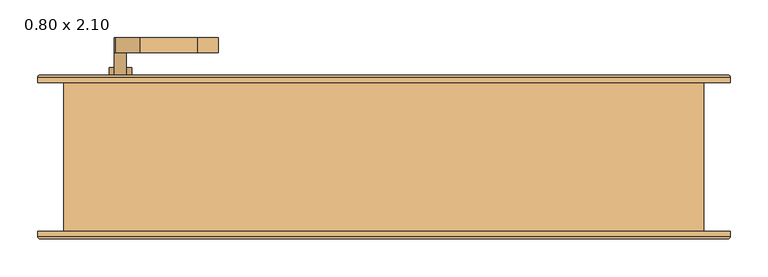
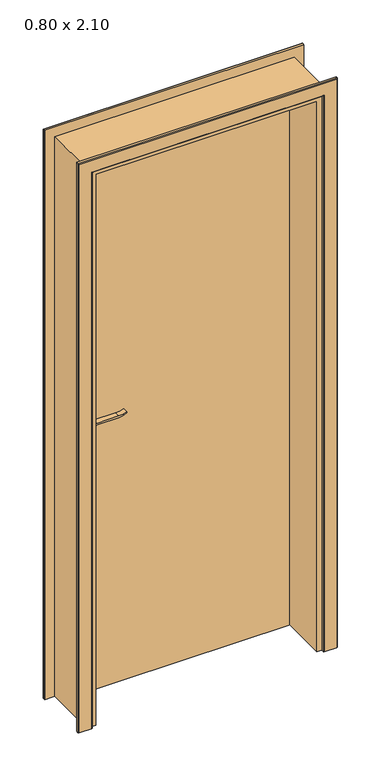
"""IFC4 building model written with IfcOpenShell, lengths in millimetres: door geometry, .CC_ND 300_PORTA SIMPLES DE ABRIR_COM EXTENSÃO : 0.80 x 2.10."""

from ifc_helpers import new_model, si_unit, point, frame, frame_2d, origin, origin_with_axes, place, context, project, spatial, polyline, circle_curve, ellipse_curve, trimmed, segment, composite_curve, outline, extrude, faceted_brep, source, transform, mapped, element, save
from ifc_brep_helpers import plane_surface, cylinder_surface, advanced_brep


def door_0_80_x_2_10_6188e507(model_context):
    return source(origin(), model_context, "Body", "SolidModel", [
        extrude(outline(composite_curve([segment(trimmed(circle_curve(frame_2d((964.5, -350.0)), 15.0), [point((964.5, -335.0))], [point((964.5, -365.0))], False, "CARTESIAN"), True, "CONTINUOUS"), segment(trimmed(circle_curve(frame_2d((964.5, -350.0)), 15.0), [point((964.5, -365.0))], [point((964.5, -335.0))], False, "CARTESIAN"), True, "CONTINUOUS")], self_intersect=False)), frame((0.0, 108.8, 0.0), z_axis=(0.0, 1.0, 0.0), x_axis=(0.0, 0.0, 1.0)), (0.0, 0.0, 1.0), 10.0),
        extrude(outline(composite_curve([segment(trimmed(circle_curve(frame_2d((964.5, -350.0)), 15.0), [point((964.5, -335.0))], [point((964.5, -365.0))], False, "CARTESIAN"), True, "CONTINUOUS"), segment(trimmed(circle_curve(frame_2d((964.5, -350.0)), 15.0), [point((964.5, -365.0))], [point((964.5, -335.0))], False, "CARTESIAN"), True, "CONTINUOUS")], self_intersect=False)), frame((0.0, 48.8, 0.0), z_axis=(0.0, 1.0, 0.0), x_axis=(0.0, 0.0, 1.0)), (0.0, 0.0, 1.0), 10.0),
        extrude(outline(composite_curve([segment(trimmed(circle_curve(frame_2d((1024.5, -350.0)), 8.0), [point((1029.1523287, -356.5081363))], [point((1024.5, -342.0))], False, "CARTESIAN"), True, "CONTINUOUS"), segment(trimmed(circle_curve(frame_2d((1019.3738613, -324.6138099)), 18.1261387), [point((1024.5, -342.0))], [point((1037.5, -324.6138099))], True, "CARTESIAN"), True, "CONTINUOUS"), segment(polyline([(1037.5, -324.6138099), (1037.5, -248.3564091)]), True, "CONTINUOUS"), segment(trimmed(circle_curve(frame_2d((1096.7709207, -251.9396612)), 59.3791355), [point((1037.5, -248.3564091))], [point((1046.7135558, -220.0))], False, "CARTESIAN"), True, "CONTINUOUS"), segment(polyline([(1046.7135558, -220.0), (1049.5, -220.0)]), True, "CONTINUOUS"), segment(trimmed(circle_curve(frame_2d((1127.7850638, -248.4227909)), 83.2850902), [point((1049.5, -220.0))], [point((1044.5, -248.3564091))], True, "CARTESIAN"), True, "CONTINUOUS"), segment(polyline([(1044.5, -248.3564091), (1044.5, -324.6325667)]), True, "CONTINUOUS"), segment(trimmed(circle_curve(frame_2d((1007.2555521, -326.3324871)), 37.2832219), [point((1044.5, -324.6325667))], [point((1029.1523287, -356.5081363))], False, "CARTESIAN"), True, "CONTINUOUS")], self_intersect=False)), frame((0.0, 138.8, 0.0), z_axis=(0.0, 1.0, 0.0), x_axis=(0.0, 0.0, 1.0)), (0.0, 0.0, 1.0), 20.0),
        extrude(outline(composite_curve([segment(trimmed(circle_curve(frame_2d((1019.3738682, -324.6138122)), 18.1261318), [point((1024.4999903, -342.0))], [point((1037.5, -324.6138122))], True, "CARTESIAN"), True, "CONTINUOUS"), segment(polyline([(1037.5, -324.6138122), (1037.5, -248.3564091)]), True, "CONTINUOUS"), segment(trimmed(circle_curve(frame_2d((1096.7709207, -251.9396612)), 59.3791355), [point((1037.5, -248.3564091))], [point((1046.7135558, -220.0))], False, "CARTESIAN"), True, "CONTINUOUS"), segment(polyline([(1046.7135558, -220.0), (1049.5, -220.0)]), True, "CONTINUOUS"), segment(trimmed(circle_curve(frame_2d((1127.7850638, -248.4227909)), 83.2850902), [point((1049.5, -220.0))], [point((1044.5, -248.3564091))], True, "CARTESIAN"), True, "CONTINUOUS"), segment(polyline([(1044.5, -248.3564091), (1044.5, -324.6325667)]), True, "CONTINUOUS"), segment(trimmed(circle_curve(frame_2d((1007.2555521, -326.3324871)), 37.2832219), [point((1044.5, -324.6325667))], [point((1029.1523287, -356.5081363))], False, "CARTESIAN"), True, "CONTINUOUS"), segment(trimmed(circle_curve(frame_2d((1024.5, -350.0)), 8.0), [point((1029.1523287, -356.5081363))], [point((1024.4999903, -342.0))], False, "CARTESIAN"), True, "CONTINUOUS")], self_intersect=False)), frame((0.0, 8.8, 0.0), z_axis=(0.0, 1.0, 0.0), x_axis=(0.0, 0.0, 1.0)), (0.0, 0.0, 1.0), 20.0),
        extrude(outline(composite_curve([segment(trimmed(circle_curve(frame_2d((1024.5, -350.0)), 8.0), [point((1024.5, -342.0))], [point((1024.5, -358.0))], False, "CARTESIAN"), True, "CONTINUOUS"), segment(trimmed(circle_curve(frame_2d((1024.5, -350.0)), 8.0), [point((1024.5, -358.0))], [point((1024.5, -342.0))], False, "CARTESIAN"), True, "CONTINUOUS")], self_intersect=False)), frame((0.0, 108.8, 0.0), z_axis=(0.0, 1.0, 0.0), x_axis=(0.0, 0.0, 1.0)), (0.0, 0.0, 1.0), 30.0),
        extrude(outline(composite_curve([segment(trimmed(circle_curve(frame_2d((1024.5, -350.0)), 8.0), [point((1024.5, -342.0))], [point((1024.5, -358.0))], False, "CARTESIAN"), True, "CONTINUOUS"), segment(trimmed(circle_curve(frame_2d((1024.5, -350.0)), 8.0), [point((1024.5, -358.0))], [point((1024.5, -342.0))], False, "CARTESIAN"), True, "CONTINUOUS")], self_intersect=False)), frame((0.0, 28.8, 0.0), z_axis=(0.0, 1.0, 0.0), x_axis=(0.0, 0.0, 1.0)), (0.0, 0.0, 1.0), 30.0),
        extrude(outline(composite_curve([segment(trimmed(circle_curve(frame_2d((954.5, -350.0)), 25.0), [point((954.5, -375.0))], [point((954.5, -325.0))], False, "CARTESIAN"), True, "CONTINUOUS"), segment(polyline([(954.5, -325.0), (1024.5, -325.0)]), True, "CONTINUOUS"), segment(trimmed(circle_curve(frame_2d((1024.5, -350.0)), 25.0), [point((1024.5, -325.0))], [point((1024.5, -375.0))], False, "CARTESIAN"), True, "CONTINUOUS"), segment(polyline([(1024.5, -375.0), (954.5, -375.0)]), True, "CONTINUOUS")], self_intersect=False)), frame((0.0, 98.8, 0.0), z_axis=(0.0, 1.0, 0.0), x_axis=(0.0, 0.0, 1.0)), (0.0, 0.0, 1.0), 10.0),
        extrude(outline(composite_curve([segment(trimmed(circle_curve(frame_2d((954.5, -350.0)), 25.0), [point((954.5, -375.0))], [point((954.5, -325.0))], False, "CARTESIAN"), True, "CONTINUOUS"), segment(polyline([(954.5, -325.0), (1024.5, -325.0)]), True, "CONTINUOUS"), segment(trimmed(circle_curve(frame_2d((1024.5, -350.0)), 25.0), [point((1024.5, -325.0))], [point((1024.5, -375.0))], False, "CARTESIAN"), True, "CONTINUOUS"), segment(polyline([(1024.5, -375.0), (954.5, -375.0)]), True, "CONTINUOUS")], self_intersect=False)), frame((0.0, 58.8, 0.0), z_axis=(0.0, 1.0, 0.0), x_axis=(0.0, 0.0, 1.0)), (0.0, 0.0, 1.0), 10.0),
        advanced_brep(
        [(-460.0, 98.8, 0.0), (-460.0, 105.8, 0.0), (-457.0, 108.8, 0.0), (-413.0, 108.8, 0.0), (-410.0, 105.8, 0.0), (-410.0, 98.8, 0.0), (-410.0, 98.8, 2085.0), (410.0, 98.8, 2085.0), (410.0, 98.8, 0.0), (460.0, 98.8, 0.0), (460.0, 98.8, 2135.0), (-460.0, 98.8, 2135.0), (-410.0, 105.8, 2085.0), (-413.0, 108.8, 2088.0), (-457.0, 108.8, 2132.0), (457.0, 108.8, 2132.0), (457.0, 108.8, 0.0), (413.0, 108.8, 0.0), (413.0, 108.8, 2088.0), (-460.0, 105.8, 2135.0), (460.0, 105.8, 0.0), (460.0, 105.8, 2135.0), (410.0, 105.8, 0.0), (410.0, 105.8, 2085.0)],
        [
            (0, 1),
            (1, 2, circle_curve(frame((-457.0, 105.8, 0.0), z_axis=(0.0, 0.0, -1.0), x_axis=(1.0, 0.0, 0.0)), 3.0)),
            (2, 3),
            (3, 4, circle_curve(frame((-413.0, 105.8, 0.0), z_axis=(0.0, 0.0, -1.0), x_axis=(1.0, 0.0, 0.0)), 3.0)),
            (4, 5),
            (5, 0),
            (5, 6),
            (6, 7),
            (7, 8),
            (8, 9),
            (9, 10),
            (10, 11),
            (11, 0),
            (4, 12),
            (12, 6),
            (3, 13),
            (13, 12, ellipse_curve(frame((-413.0, 105.8, 2088.0), z_axis=(-0.7071067811865475, 0.0, -0.7071067811865475), x_axis=(0.7071067811865474, 0.0, -0.7071067811865476)), 4.2426407, 3.0)),
            (2, 14),
            (14, 15),
            (15, 16),
            (16, 17),
            (17, 18),
            (18, 13),
            (1, 19),
            (19, 14, ellipse_curve(frame((-457.0, 105.8, 2132.0), z_axis=(-0.7071067811865475, 0.0, -0.7071067811865475), x_axis=(0.7071067811865474, 0.0, -0.7071067811865476)), 4.2426407, 3.0)),
            (11, 19),
            (9, 20),
            (20, 21),
            (21, 10),
            (8, 22),
            (22, 17, circle_curve(frame((413.0, 105.8, 0.0), z_axis=(0.0, 0.0, -1.0), x_axis=(-1.0, 0.0, 0.0)), 3.0)),
            (16, 20, circle_curve(frame((457.0, 105.8, 0.0), z_axis=(0.0, 0.0, -1.0), x_axis=(-1.0, 0.0, 0.0)), 3.0)),
            (23, 22),
            (7, 23),
            (23, 18, ellipse_curve(frame((413.0, 105.8, 2088.0), z_axis=(0.7071067811865475, 0.0, -0.7071067811865475), x_axis=(0.7071067811865474, 0.0, 0.7071067811865476)), 4.2426407, 3.0)),
            (15, 21, ellipse_curve(frame((457.0, 105.8, 2132.0), z_axis=(0.7071067811865475, 0.0, -0.7071067811865475), x_axis=(0.7071067811865474, 0.0, 0.7071067811865476)), 4.2426407, 3.0)),
            (12, 23),
            (21, 19),
        ],
        [
            plane_surface(frame((-410.0, 98.8, 0.0), z_axis=(0.0, 0.0, -1.0), x_axis=(0.0, -1.0, 0.0))),
            plane_surface(frame((-460.0, 98.8, 0.0), z_axis=(0.0, -1.0, 0.0), x_axis=(0.0, 0.0, 1.0))),
            plane_surface(frame((-410.0, 98.8, 0.0), z_axis=(1.0, 0.0, 0.0), x_axis=(0.0, 0.0, 1.0))),
            cylinder_surface(frame((-413.0, 105.8, 0.0), z_axis=(0.0, 0.0, -1.0), x_axis=(1.0, 0.0, 0.0)), 3.0),
            plane_surface(frame((-413.0, 108.8, 0.0), z_axis=(0.0, 1.0, 0.0), x_axis=(0.0, 0.0, 1.0))),
            cylinder_surface(frame((-457.0, 105.8, 0.0), z_axis=(0.0, 0.0, -1.0), x_axis=(1.0, 0.0, 0.0)), 3.0),
            plane_surface(frame((-460.0, 105.8, 0.0), z_axis=(-1.0, 0.0, 0.0), x_axis=(0.0, 0.0, 1.0))),
            plane_surface(frame((460.0, 105.8, 2135.0), z_axis=(1.0, 0.0, 0.0), x_axis=(0.0, 0.0, -1.0))),
            plane_surface(frame((410.0, 98.8, 0.0), z_axis=(0.0, 0.0, -1.0), x_axis=(0.0, -1.0, 0.0))),
            plane_surface(frame((410.0, 98.8, 2085.0), z_axis=(-1.0, 0.0, 0.0), x_axis=(0.0, 0.0, -1.0))),
            cylinder_surface(frame((413.0, 105.8, 2085.0), z_axis=(0.0, 0.0, 1.0), x_axis=(-1.0, 0.0, 0.0)), 3.0),
            cylinder_surface(frame((457.0, 105.8, 2085.0), z_axis=(0.0, 0.0, 1.0), x_axis=(-1.0, 0.0, 0.0)), 3.0),
            plane_surface(frame((-410.0, 98.8, 2085.0), z_axis=(0.0, 0.0, -1.0), x_axis=(1.0, 0.0, 0.0))),
            plane_surface(frame((-460.0, 105.8, 2135.0), z_axis=(0.0, 0.0, 1.0), x_axis=(1.0, 0.0, 0.0))),
            cylinder_surface(frame((-410.0, 105.8, 2088.0), z_axis=(-1.0, 0.0, 0.0), x_axis=(0.0, 0.0, -1.0)), 3.0),
            cylinder_surface(frame((-410.0, 105.8, 2132.0), z_axis=(-1.0, 0.0, 0.0), x_axis=(0.0, 0.0, -1.0)), 3.0),
        ],
        [
            (0, [[1, 2, 3, 4, 5, 6]]),
            (1, [[7, 8, 9, 10, 11, 12, 13, -6]]),
            (2, [[14, 15, -7, -5]]),
            (3, [[16, 17, -14, -4]]),
            (4, [[18, 19, 20, 21, 22, 23, -16, -3]]),
            (5, [[24, 25, -18, -2]]),
            (6, [[-13, 26, -24, -1]]),
            (7, [[-11, 27, 28, 29]]),
            (8, [[-10, 30, 31, -21, 32, -27]]),
            (9, [[33, -30, -9, 34]]),
            (10, [[-22, -31, -33, 35]]),
            (11, [[-28, -32, -20, 36]]),
            (12, [[37, -34, -8, -15]]),
            (13, [[-12, -29, 38, -26]]),
            (14, [[-23, -35, -37, -17]]),
            (15, [[-38, -36, -19, -25]]),
        ],
    ),
        advanced_brep(
        [(460.0, -98.8, 0.0), (460.0, -105.8342217, 0.0), (457.0342217, -108.8, 0.0), (412.9842717, -108.8, 0.0), (410.0, -105.8157283, 0.0), (410.0, -98.8, 0.0), (410.0, -98.8, 2085.0), (-410.0, -98.8, 2085.0), (-410.0, -98.8, 0.0), (-460.0, -98.8, 0.0), (-460.0, -98.8, 2135.0), (460.0, -98.8, 2135.0), (410.0, -105.8157283, 2085.0), (412.9842717, -108.8, 2087.9842717), (457.0342217, -108.8, 2132.0342217), (-457.0342217, -108.8, 2132.0342217), (-457.0342217, -108.8, 0.0), (-412.9842717, -108.8, 0.0), (-412.9842717, -108.8, 2087.9842717), (460.0, -105.8342217, 2135.0), (-460.0, -105.8342217, 0.0), (-460.0, -105.8342217, 2135.0), (-410.0, -105.8157283, 0.0), (-410.0, -105.8157283, 2085.0)],
        [
            (0, 1),
            (1, 2, circle_curve(frame((457.0342217, -105.8342217, 0.0), z_axis=(0.0, 0.0, -1.0), x_axis=(1.0, 0.0, 0.0)), 2.9657783)),
            (2, 3),
            (3, 4, circle_curve(frame((412.9842717, -105.8157283, 0.0), z_axis=(0.0, 0.0, -1.0), x_axis=(1.0, 0.0, 0.0)), 2.9842717)),
            (4, 5),
            (5, 0),
            (5, 6),
            (6, 7),
            (7, 8),
            (8, 9),
            (9, 10),
            (10, 11),
            (11, 0),
            (4, 12),
            (12, 6),
            (3, 13),
            (13, 12, ellipse_curve(frame((412.9842717, -105.8157283, 2087.9842717), z_axis=(0.7071067811865475, 0.0, -0.7071067811865475), x_axis=(-0.7071067811865474, 0.0, -0.7071067811865476)), 4.2203975, 2.9842717)),
            (2, 14),
            (14, 15),
            (15, 16),
            (16, 17),
            (17, 18),
            (18, 13),
            (1, 19),
            (19, 14, ellipse_curve(frame((457.0342217, -105.8342217, 2132.0342217), z_axis=(0.7071067811865475, 0.0, -0.7071067811865475), x_axis=(-0.7071067811865474, 0.0, -0.7071067811865476)), 4.1942438, 2.9657783)),
            (11, 19),
            (9, 20),
            (20, 21),
            (21, 10),
            (8, 22),
            (22, 17, circle_curve(frame((-412.9842717, -105.8157283, 0.0), z_axis=(0.0, 0.0, -1.0), x_axis=(-1.0, 0.0, 0.0)), 2.9842717)),
            (16, 20, circle_curve(frame((-457.0342217, -105.8342217, 0.0), z_axis=(0.0, 0.0, -1.0), x_axis=(-1.0, 0.0, 0.0)), 2.9657783)),
            (23, 22),
            (7, 23),
            (23, 18, ellipse_curve(frame((-412.9842717, -105.8157283, 2087.9842717), z_axis=(-0.7071067811865475, 0.0, -0.7071067811865475), x_axis=(-0.7071067811865474, 0.0, 0.7071067811865476)), 4.2203975, 2.9842717)),
            (15, 21, ellipse_curve(frame((-457.0342217, -105.8342217, 2132.0342217), z_axis=(-0.7071067811865475, 0.0, -0.7071067811865475), x_axis=(-0.7071067811865474, 0.0, 0.7071067811865476)), 4.1942438, 2.9657783)),
            (12, 23),
            (21, 19),
        ],
        [
            plane_surface(frame((410.0, -98.8, 0.0), z_axis=(0.0, 0.0, -1.0), x_axis=(0.0, -1.0, 0.0))),
            plane_surface(frame((460.0, -98.8, 0.0), z_axis=(0.0, 1.0, 0.0), x_axis=(0.0, 0.0, 1.0))),
            plane_surface(frame((410.0, -98.8, 0.0), z_axis=(-1.0, 0.0, 0.0), x_axis=(0.0, 0.0, 1.0))),
            cylinder_surface(frame((412.9842717, -105.8157283, 0.0), z_axis=(0.0, 0.0, -1.0), x_axis=(1.0, 0.0, 0.0)), 2.9842717),
            plane_surface(frame((412.9842717, -108.8, 0.0), z_axis=(0.0, -1.0, 0.0), x_axis=(0.0, 0.0, 1.0))),
            cylinder_surface(frame((457.0342217, -105.8342217, 0.0), z_axis=(0.0, 0.0, -1.0), x_axis=(1.0, 0.0, 0.0)), 2.9657783),
            plane_surface(frame((460.0, -105.8342217, 0.0), z_axis=(1.0, 0.0, 0.0), x_axis=(0.0, 0.0, 1.0))),
            plane_surface(frame((-460.0, -105.8342217, 2135.0), z_axis=(-1.0, 0.0, 0.0), x_axis=(0.0, 0.0, -1.0))),
            plane_surface(frame((-410.0, -98.8, 0.0), z_axis=(0.0, 0.0, -1.0), x_axis=(0.0, -1.0, 0.0))),
            plane_surface(frame((-410.0, -98.8, 2085.0), z_axis=(1.0, 0.0, 0.0), x_axis=(0.0, 0.0, -1.0))),
            cylinder_surface(frame((-412.9842717, -105.8157283, 2085.0), z_axis=(0.0, 0.0, 1.0), x_axis=(-1.0, 0.0, 0.0)), 2.9842717),
            cylinder_surface(frame((-457.0342217, -105.8342217, 2085.0), z_axis=(0.0, 0.0, 1.0), x_axis=(-1.0, 0.0, 0.0)), 2.9657783),
            plane_surface(frame((410.0, -98.8, 2085.0), z_axis=(0.0, 0.0, -1.0), x_axis=(-1.0, 0.0, 0.0))),
            plane_surface(frame((460.0, -105.8342217, 2135.0), z_axis=(0.0, 0.0, 1.0), x_axis=(-1.0, 0.0, 0.0))),
            cylinder_surface(frame((410.0, -105.8157283, 2087.9842717), z_axis=(1.0, 0.0, 0.0), x_axis=(0.0, 0.0, 1.0)), 2.9842717),
            cylinder_surface(frame((410.0, -105.8342217, 2132.0342217), z_axis=(1.0, 0.0, 0.0), x_axis=(0.0, 0.0, 1.0)), 2.9657783),
        ],
        [
            (0, [[1, 2, 3, 4, 5, 6]]),
            (1, [[7, 8, 9, 10, 11, 12, 13, -6]]),
            (2, [[14, 15, -7, -5]]),
            (3, [[16, 17, -14, -4]]),
            (4, [[18, 19, 20, 21, 22, 23, -16, -3]]),
            (5, [[24, 25, -18, -2]]),
            (6, [[-13, 26, -24, -1]]),
            (7, [[-11, 27, 28, 29]]),
            (8, [[-10, 30, 31, -21, 32, -27]]),
            (9, [[33, -30, -9, 34]]),
            (10, [[-22, -31, -33, 35]]),
            (11, [[-28, -32, -20, 36]]),
            (12, [[37, -34, -8, -15]]),
            (13, [[-12, -29, 38, -26]]),
            (14, [[-23, -35, -37, -17]]),
            (15, [[-38, -36, -19, -25]]),
        ],
    ),
        faceted_brep([(392.0, -98.8, 0.0), (392.0, 68.8, 0.0), (400.0, 68.8, 0.0), (400.0, 98.8, 0.0), (425.0, 98.8, 0.0), (425.0, -98.8, 0.0), (425.0, -98.8, 2100.0), (-425.0, -98.8, 2100.0), (-425.0, -98.8, 0.0), (-392.0, -98.8, 0.0), (-392.0, -98.8, 2067.0), (392.0, -98.8, 2067.0), (425.0, 98.8, 2100.0), (400.0, 98.8, 2075.0), (-400.0, 98.8, 2075.0), (-400.0, 98.8, 0.0), (-425.0, 98.8, 0.0), (-425.0, 98.8, 2100.0), (400.0, 68.8, 2075.0), (392.0, 68.8, 2067.0), (-392.0, 68.8, 2067.0), (-392.0, 68.8, 0.0), (-400.0, 68.8, 0.0), (-400.0, 68.8, 2075.0)], [[[0, 1, 2, 3, 4, 5]], [[5, 6, 7, 8, 9, 10, 11, 0]], [[4, 12, 6, 5]], [[3, 13, 14, 15, 16, 17, 12, 4]], [[2, 18, 13, 3]], [[1, 19, 20, 21, 22, 23, 18, 2]], [[0, 11, 19, 1]], [[10, 9, 21, 20]], [[9, 8, 16, 15, 22, 21]], [[17, 16, 8, 7]], [[23, 22, 15, 14]], [[12, 17, 7, 6]], [[18, 23, 14, 13]], [[11, 10, 20, 19]]]),
        extrude(outline(polyline([(-400.0, 68.8), (-400.0, 98.8), (400.0, 98.8), (400.0, 68.8), (-400.0, 68.8)])), origin_with_axes(), (0.0, 0.0, 1.0), 2075.0),
    ])


if __name__ == "__main__":
    model = new_model("IFC4")
    model_context = context("Model", 3, world=origin())
    ifc_project = project(units=[si_unit("LENGTHUNIT", "METRE", prefix="MILLI")], contexts=[model_context])
    site = spatial("IfcSite", under=ifc_project)
    building = spatial("IfcBuilding", under=site)
    placement = place(None, origin())
    door_0_80_x_2_10_shape = door_0_80_x_2_10_6188e507(model_context)
    element("IfcDoor", 1, ObjectType=".CC_ND 300_PORTA SIMPLES DE ABRIR_COM EXTENSÃO : 0.80 x 2.10", at=placement, inside=building, context=model_context, shape_type="MappedRepresentation", body=[
        mapped(door_0_80_x_2_10_shape, transform((0.0, 0.0, 0.0), x_axis=(1.0, 0.0, 0.0), y_axis=(0.0, 1.0, 0.0), z_axis=(0.0, 0.0, 1.0))),
    ])
    save(model, "model.ifc")

# Revit data of these elements
# Type ".CC_ND 300_PORTA SIMPLES DE ABRIR_COM EXTENSÃO : 0.80 x 2.10"
#   Type Mark = "153"
#   Rough Width = 0.85 m
#   Espessura moldura externa = 0.01 m
#   Espessura moldura interna = 0.01 m
#   Largura moldura = 0.05 m
#   Extensão acabamento exterior [instance default] = 0.00 m
#   Extensão acabamento interior [instance default] = 0.00 m
#   Espessura batente = 0.025 m
#   Thickness = 0.03 m
#   Altura batente = 2.085 m
#   Aux Arco [instance default] = 0.80 m
#   Rough Height = 2.125 m
#   Height = 2.10 m
#   Width = 0.80 m
#   Moldura interna [instance default] = yes
#   Moldura externa [instance default] = yes
#   Porta = .MADEIRA COM PINTURA ESMALTE BRANCO ACETINADO
#   Moldura = .MADEIRA COM PINTURA ESMALTE BRANCO ACETINADO
#   Maçaneta = .ALUMÍNIO
#   Batente = .MADEIRA COM PINTURA ESMALTE BRANCO ACETINADO
#   Function = (empty or 0)
#   Wall Closure = (empty or 0)
# Element 1 (IfcDoor, ".CC_ND 300_PORTA SIMPLES DE ABRIR_COM EXTENSÃO : 0.80 x 2.10")
#   Materials on its faces: ".MADEIRA COM PINTURA ESMALTE BRANCO ACETINADO", ".ALUMÍNIO"
# Materials
#   ".MADEIRA COM PINTURA ESMALTE BRANCO ACETINADO": class ".CC_MADEIRAS", colour RGB 240 240 240, transparency 0, Description = "Madeira com pintura esmalte branco acetinado.", Cost = 0
#   ".ALUMÍNIO": class "CC_METAIS", colour RGB 244 244 244, transparency 0, Description = "Material alumínio", Cost = 0
